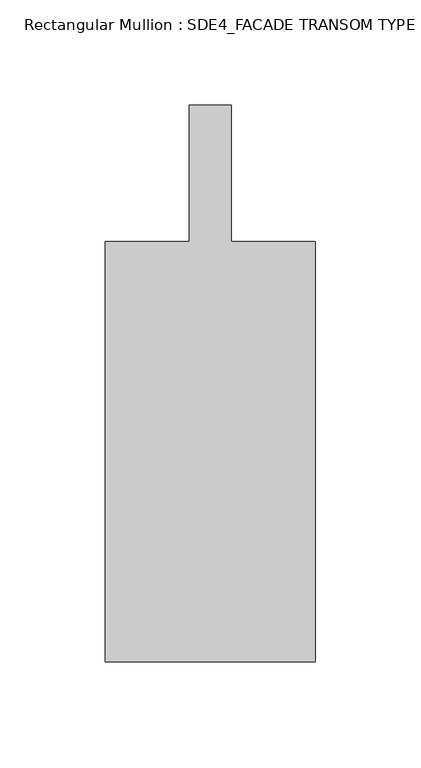
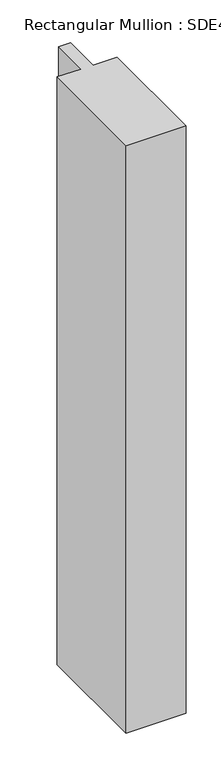
"""IFC4 building model written with IfcOpenShell, lengths in millimetres: member geometry, Rectangular Mullion : SDE4_FACADE TRANSOM TYPE 2."""

from ifc_helpers import new_model, si_unit, frame, origin, place, context, project, spatial, polyline, outline, extrude, source, transform, mapped, element, save


def rectangular_mullion_sde4_facade_transom_type_2_651ea07a(model_context):
    return source(origin(), model_context, "Body", "SweptSolid", [
        extrude(outline(polyline([(50.0, -132.5), (-50.0, -132.5), (-50.0, 67.5), (-10.0, 67.5), (-10.0, 132.5), (10.0, 132.5), (10.0, 67.5), (50.0, 67.5), (50.0, -132.5)])), frame((0.0, 0.0, -1039.0000004), z_axis=(0.0, 0.0, 1.0), x_axis=(1.0, 0.0, 0.0)), (0.0, 0.0, 1.0), 1039.0000004),
    ])


if __name__ == "__main__":
    model = new_model("IFC4")
    model_context = context("Model", 3, world=origin())
    ifc_project = project(units=[si_unit("LENGTHUNIT", "METRE", prefix="MILLI")], contexts=[model_context])
    site = spatial("IfcSite", under=ifc_project)
    building = spatial("IfcBuilding", under=site)
    placement = place(None, origin())
    rectangular_mullion_sde4_facade_transom_type_2_shape = rectangular_mullion_sde4_facade_transom_type_2_651ea07a(model_context)
    element("IfcMember", 1, ObjectType="Rectangular Mullion : SDE4_FACADE TRANSOM TYPE 2", at=placement, inside=building, context=model_context, shape_type="MappedRepresentation", body=[
        mapped(rectangular_mullion_sde4_facade_transom_type_2_shape, transform((0.0, 0.0, 0.0), x_axis=(1.0, 0.0, 0.0), y_axis=(0.0, 1.0, 0.0), z_axis=(0.0, 0.0, 1.0))),
    ])
    save(model, "model.ifc")

# Revit data of these elements
# Type "Rectangular Mullion : SDE4_FACADE TRANSOM TYPE 2"
#   built-in parameter 1007322 = 0.869423 (stored number, unit not read)
#   built-in parameter 1007321 = 0.164042 (stored number, unit not read)
#   built-in parameter 1007320 = 0.164042 (stored number, unit not read)
